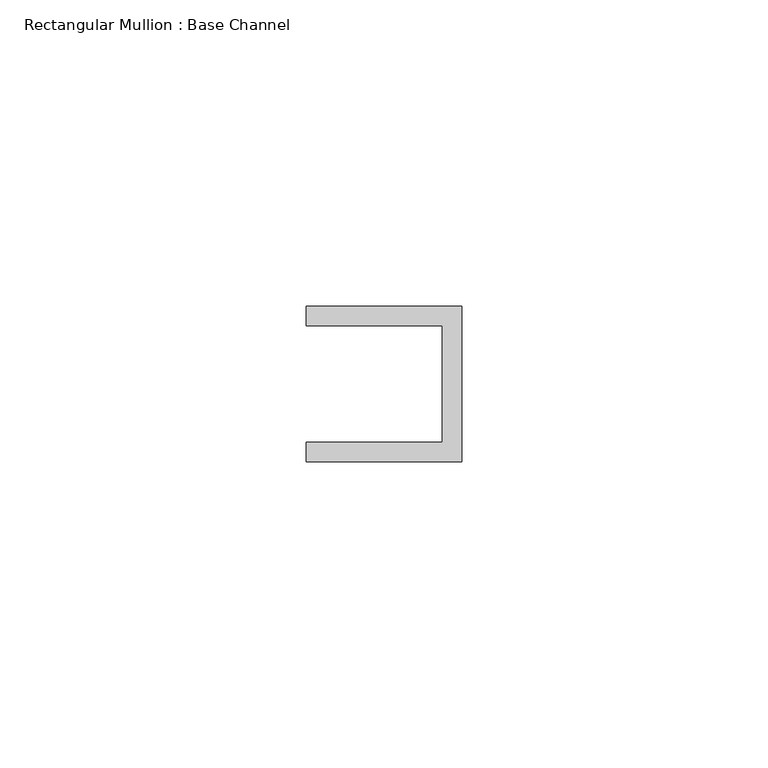
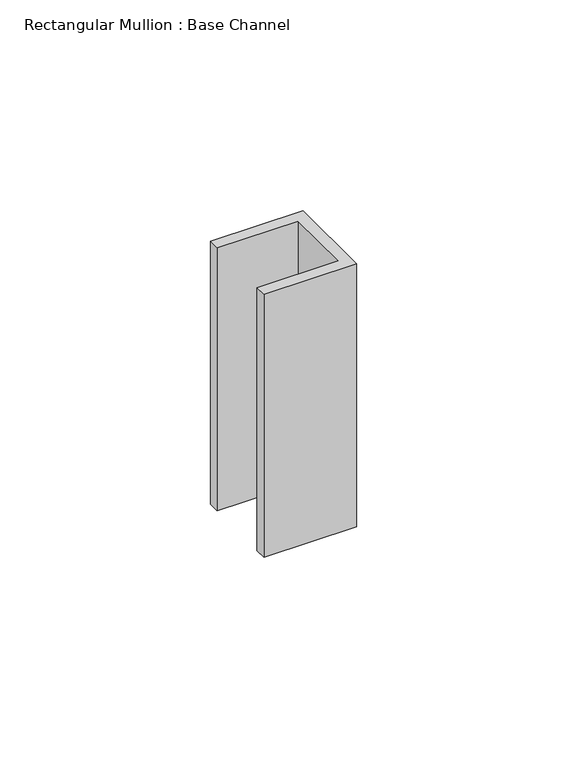
"""IFC4 building model written with IfcOpenShell, lengths in millimetres: member geometry, Rectangular Mullion : Base Channel."""

from ifc_helpers import new_model, si_unit, frame, origin, place, context, project, spatial, polyline, outline, extrude, source, transform, mapped, element, save


def rectangular_mullion_base_channel_fd5d5daf(model_context):
    return source(origin(), model_context, "Body", "SweptSolid", [
        extrude(outline(polyline([(0.0, 12.7), (0.0, -12.7), (-25.4, -12.7), (-25.4, -9.525), (-3.175, -9.525), (-3.175, 9.525), (-25.4, 9.525), (-25.4, 12.7), (0.0, 12.7)])), frame((0.0, 0.0, -76.2), z_axis=(0.0, 0.0, 1.0), x_axis=(1.0, 0.0, 0.0)), (0.0, 0.0, 1.0), 76.2),
    ])


if __name__ == "__main__":
    model = new_model("IFC4")
    model_context = context("Model", 3, world=origin())
    ifc_project = project(units=[si_unit("LENGTHUNIT", "METRE", prefix="MILLI")], contexts=[model_context])
    site = spatial("IfcSite", under=ifc_project)
    building = spatial("IfcBuilding", under=site)
    placement = place(None, origin())
    rectangular_mullion_base_channel_shape = rectangular_mullion_base_channel_fd5d5daf(model_context)
    element("IfcMember", 1, ObjectType="Rectangular Mullion : Base Channel", at=placement, inside=building, context=model_context, shape_type="MappedRepresentation", body=[
        mapped(rectangular_mullion_base_channel_shape, transform((0.0, 0.0, 0.0), x_axis=(1.0, 0.0, 0.0), y_axis=(0.0, 1.0, 0.0), z_axis=(0.0, 0.0, 1.0))),
    ])
    save(model, "model.ifc")

# Revit data of these elements
# Type "Rectangular Mullion : Base Channel"
#   built-in parameter 1007322 = 0.0833333 (stored number, unit not read)
#   built-in parameter 1007321 = 0.0416667 (stored number, unit not read)
#   built-in parameter 1007320 = -0.03125 (stored number, unit not read)
# Element 1 (IfcMember, "Rectangular Mullion : Base Channel")
#   Materials on its faces: "ALUM"
# Materials
#   "ALUM": class "Generic", colour RGB 157 157 157, transparency 0, Cost = 0
